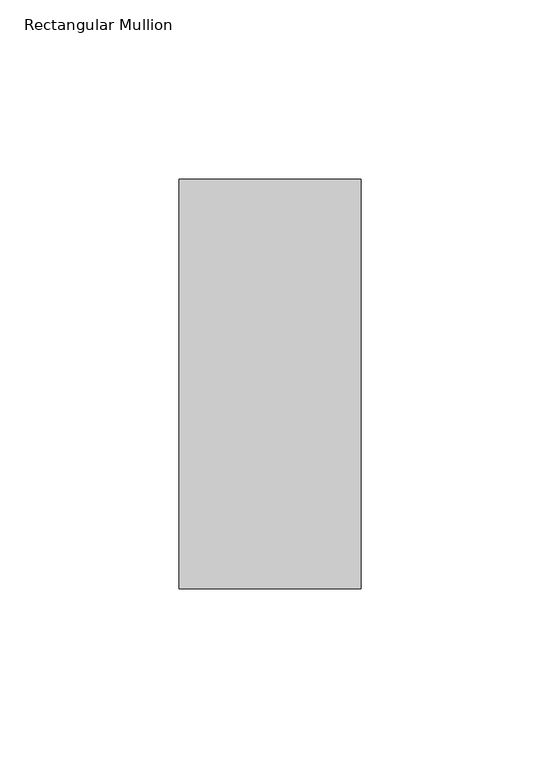
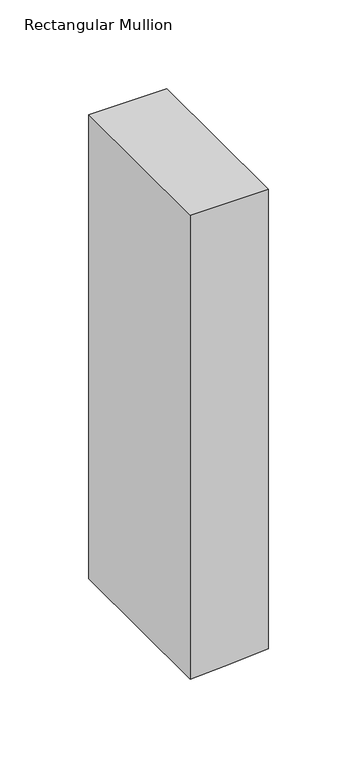
"""IFC4 building model written with IfcOpenShell, lengths in millimetres: member geometry, Rectangular Mullion : KAWNEER TRIFAB VERSAGLAZE 451T - CLEAR ANODIZED ALUM. - BACK GLAZED."""

from ifc_helpers import new_model, si_unit, frame, origin, place, context, project, spatial, polyline, outline, extrude, source, transform, mapped, element, save


def rectangular_mullion_8a0e7974(model_context):
    return source(origin(), model_context, "Body", "SweptSolid", [
        extrude(outline(polyline([(0.0, 25.4), (0.0, -25.4), (-319.4844717, -25.4), (-318.0950228, -3.1688169), (-316.3094717, 25.4), (0.0, 25.4)])), frame((0.0, -57.15, 0.0), z_axis=(0.0, 1.0, 0.0), x_axis=(0.0, 0.0, 1.0)), (0.0, 0.0, 1.0), 114.3),
    ])


if __name__ == "__main__":
    model = new_model("IFC4")
    model_context = context("Model", 3, world=origin())
    ifc_project = project(units=[si_unit("LENGTHUNIT", "METRE", prefix="MILLI")], contexts=[model_context])
    site = spatial("IfcSite", under=ifc_project)
    building = spatial("IfcBuilding", under=site)
    placement = place(None, origin())
    rectangular_mullion_shape = rectangular_mullion_8a0e7974(model_context)
    element("IfcMember", 1, ObjectType="Rectangular Mullion : KAWNEER TRIFAB VERSAGLAZE 451T - CLEAR ANODIZED ALUM. - BACK GLAZED", at=placement, inside=building, context=model_context, shape_type="MappedRepresentation", body=[
        mapped(rectangular_mullion_shape, transform((0.0, 0.0, 0.0), x_axis=(1.0, 0.0, 0.0), y_axis=(0.0, 1.0, 0.0), z_axis=(0.0, 0.0, 1.0))),
    ])
    save(model, "model.ifc")

# Revit data of these elements
# Type "Rectangular Mullion : KAWNEER TRIFAB VERSAGLAZE 451T - CLEAR ANODIZED ALUM. - BACK GLAZED"
#   built-in parameter 1007304 = 0.375 (stored number, unit not read)
#   built-in parameter 1007301 = 0.0833333 (stored number, unit not read)
#   built-in parameter 1007300 = 0.0833333 (stored number, unit not read)
# Element 1 (IfcMember, "Rectangular Mullion : KAWNEER TRIFAB VERSAGLAZE 451T - CLEAR ANODIZED ALUM. - BACK GLAZED")
#   Materials on its faces: "KAWNEER TRIFAB VERSAGLAZE 451T - CLEAR ANODIZED ALUM. - BACK GLAZED"
# Materials
#   "KAWNEER TRIFAB VERSAGLAZE 451T - CLEAR ANODIZED ALUM. - BACK GLAZED": class "Metal", colour RGB 244 244 244, transparency 0, Description = "Aluminum 6061", Cost = 0
